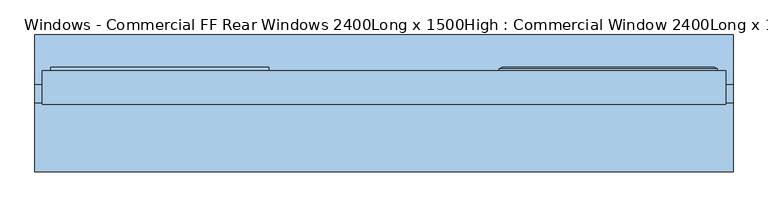
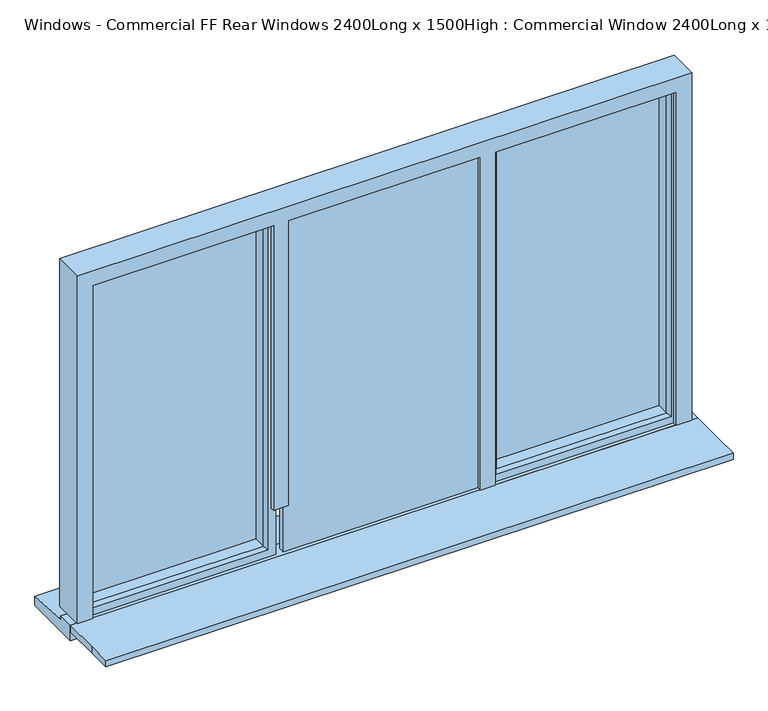
"""IFC4 building model written with IfcOpenShell, lengths in millimetres: window geometry, Windows - Commercial FF Rear Windows 2400Long x 1500High : Commercial Window 2400Long x 1500High."""

from ifc_helpers import new_model, si_unit, frame, origin, place, context, project, spatial, polyline, outline, extrude, faceted_brep, source, transform, mapped, element, save


def windows_commercial_ff_rear_windows_2400long_x_1500high_d88e899e(model_context):
    return source(origin(), model_context, "Body", "SolidModel", [
        extrude(outline(polyline([(-1860.0, -231.5434322), (-1860.0, -138.5434322), (-1860.0, 8.4565678), (590.0, 8.4565678), (590.0, -138.5434322), (590.0, -231.5434322), (-1860.0, -231.5434322)])), frame((0.0, 0.0, 636.5715519), z_axis=(0.0, 0.0, 1.0), x_axis=(1.0, 0.0, 0.0)), (0.0, 0.0, 1.0), 26.4284481),
        extrude(outline(polyline([(495.0, 87.4565678), (-190.0, 87.4565678), (-190.0, 111.4565678), (495.0, 111.4565678), (495.0, 87.4565678)])), frame((0.0, 0.0, 693.0), z_axis=(0.0, 0.0, 1.0), x_axis=(1.0, 0.0, 0.0)), (0.0, 0.0, 1.0), 1337.0),
        extrude(outline(polyline([(-1020.0, 47.4565678), (-250.0, 47.4565678), (-250.0, 23.4565678), (-1020.0, 23.4565678), (-1020.0, 47.4565678)])), frame((0.0, 0.0, 663.0), z_axis=(0.0, 0.0, 1.0), x_axis=(1.0, 0.0, 0.0)), (0.0, 0.0, 1.0), 1397.0),
        extrude(outline(polyline([(-1080.0, 87.4565678), (-1765.0, 87.4565678), (-1765.0, 111.4565678), (-1080.0, 111.4565678), (-1080.0, 87.4565678)])), frame((0.0, 0.0, 693.0), z_axis=(0.0, 0.0, 1.0), x_axis=(1.0, 0.0, 0.0)), (0.0, 0.0, 1.0), 1337.0),
        faceted_brep([(-1835.0, 5.4565678, 663.0), (-1775.0, 5.4565678, 663.0), (-1775.0, 5.4565678, 2040.0), (-1068.0, 5.4565678, 2040.0), (-1068.0, 5.4565678, 863.0), (-1010.0, 5.4565678, 863.0), (-1010.0, 5.4565678, 2040.0), (-260.0, 5.4565678, 2040.0), (-260.0, 5.4565678, 663.0), (-202.0, 5.4565678, 663.0), (-202.0, 5.4565678, 2040.0), (505.0, 5.4565678, 2040.0), (505.0, 5.4565678, 663.0), (565.0, 5.4565678, 663.0), (565.0, 5.4565678, 2100.0), (-1835.0, 5.4565678, 2100.0), (-1835.0, 123.4565678, 2100.0), (-1835.0, 123.4565678, 663.0), (-1835.0, 73.4565678, 663.0), (-1835.0, 8.4565678, 663.0), (-1795.0, 123.4565678, 663.0), (565.0, 123.4565678, 2100.0), (565.0, 123.4565678, 663.0), (525.0, 123.4565678, 663.0), (525.0, 123.4565678, 2060.0), (-220.0, 123.4565678, 2060.0), (-220.0, 123.4565678, 663.0), (-260.0, 123.4565678, 663.0), (-260.0, 123.4565678, 2060.0), (-1010.0, 123.4565678, 2060.0), (-1010.0, 123.4565678, 863.0), (-1050.0, 123.4565678, 863.0), (-1050.0, 123.4565678, 2060.0), (-1795.0, 123.4565678, 2060.0), (-1795.0, 23.4565678, 2060.0), (-1795.0, 23.4565678, 663.0), (-1795.0, 73.4565678, 663.0), (-1050.0, 23.4565678, 2060.0), (-1050.0, 23.4565678, 863.0), (-1068.0, 23.4565678, 863.0), (-1068.0, 23.4565678, 2040.0), (-1775.0, 23.4565678, 2040.0), (-1775.0, 23.4565678, 663.0), (525.0, 23.4565678, 2060.0), (525.0, 23.4565678, 663.0), (505.0, 23.4565678, 663.0), (505.0, 23.4565678, 2040.0), (-202.0, 23.4565678, 2040.0), (-202.0, 23.4565678, 663.0), (-220.0, 23.4565678, 663.0), (-220.0, 23.4565678, 2060.0), (-1010.0, 23.4565678, 863.0), (-1020.0, 23.4565678, 863.0), (-1020.0, 23.4565678, 2060.0), (-250.0, 23.4565678, 2060.0), (-250.0, 23.4565678, 663.0), (-260.0, 23.4565678, 663.0), (-260.0, 23.4565678, 2040.0), (-1010.0, 23.4565678, 2040.0), (-1775.0, 8.4565678, 663.0), (-1010.0, 47.4565678, 2060.0), (-260.0, 47.4565678, 2060.0), (-250.0, 47.4565678, 2060.0), (-1020.0, 47.4565678, 2060.0), (565.0, 8.4565678, 663.0), (565.0, 73.4565678, 663.0), (525.0, 73.4565678, 663.0), (505.0, 8.4565678, 663.0), (-1010.0, 47.4565678, 863.0), (-1020.0, 47.4565678, 863.0), (-250.0, 47.4565678, 663.0), (-260.0, 47.4565678, 663.0), (-260.0, 73.4565678, 663.0), (-220.0, 73.4565678, 663.0), (-202.0, 8.4565678, 663.0), (-260.0, 8.4565678, 663.0), (590.0, 248.4565678, 600.0), (590.0, 8.4565678, 600.0), (-1860.0, 8.4565678, 600.0), (-1860.0, 248.4565678, 600.0), (590.0, 248.4565678, 637.0666405), (-1860.0, 248.4565678, 637.0666405), (590.0, 73.4565678, 649.0962075), (-1860.0, 73.4565678, 649.0962075), (590.0, 8.4565678, 663.0), (590.0, 73.4565678, 663.0), (-1860.0, 73.4565678, 663.0), (-1860.0, 8.4565678, 663.0)], [[[0, 1, 2, 3, 4, 5, 6, 7, 8, 9, 10, 11, 12, 13, 14, 15]], [[0, 15, 16, 17, 18, 19]], [[20, 17, 16, 21, 22, 23, 24, 25, 26, 27, 28, 29, 30, 31, 32, 33]], [[20, 33, 34, 35, 36]], [[35, 34, 37, 38, 39, 40, 41, 42]], [[43, 44, 45, 46, 47, 48, 49, 50]], [[51, 52, 53, 54, 55, 56, 57, 58]], [[2, 1, 59, 42, 41]], [[15, 14, 21, 16]], [[34, 33, 32, 37]], [[24, 43, 50, 25]], [[60, 29, 28, 61, 62, 54, 53, 63]], [[2, 41, 40, 3]], [[46, 11, 10, 47]], [[6, 58, 57, 7]], [[14, 13, 64, 65, 22, 21]], [[24, 23, 66, 44, 43]], [[12, 11, 46, 45, 67]], [[5, 51, 58, 6]], [[39, 4, 3, 40]], [[31, 38, 37, 32]], [[68, 30, 29, 60]], [[69, 68, 60, 63]], [[52, 69, 63, 53]], [[62, 70, 55, 54]], [[70, 62, 61, 71]], [[71, 61, 28, 27, 72]], [[26, 25, 50, 49, 73]], [[10, 9, 74, 48, 47]], [[8, 7, 57, 56, 75]], [[76, 77, 78, 79]], [[80, 76, 79, 81]], [[82, 80, 81, 83]], [[84, 85, 65, 64]], [[86, 87, 19, 18]], [[72, 36, 35, 42, 59, 75, 56, 55, 70, 71]], [[66, 73, 49, 48, 74, 67, 45, 44]], [[17, 20, 36, 18]], [[1, 0, 19, 59]], [[23, 22, 65, 66]], [[13, 12, 67, 64]], [[51, 5, 4, 39, 38, 31, 30, 68, 69, 52]], [[27, 26, 73, 72]], [[9, 8, 75, 74]], [[84, 77, 76, 80, 82, 85]], [[87, 86, 83, 81, 79, 78]], [[85, 82, 83, 86, 18, 36, 72, 73, 66, 65]], [[77, 84, 64, 67, 74, 75, 59, 19, 87, 78]]]),
        faceted_brep([(-1050.0, 23.4565678, 2060.0), (-1050.0, 93.4565678, 2060.0), (-1795.0, 93.4565678, 2060.0), (-1795.0, 23.4565678, 2060.0), (-1090.0, 37.9494677, 2020.0), (-1079.8519623, 23.4565678, 2030.1480377), (-1765.1480377, 23.4565678, 2030.1480377), (-1755.0, 37.9494677, 2020.0), (-1090.0, 87.4565678, 2020.0), (-1755.0, 87.4565678, 2020.0), (-1080.0, 111.4565678, 2030.0), (-1080.0, 87.4565678, 2030.0), (-1765.0, 87.4565678, 2030.0), (-1765.0, 111.4565678, 2030.0), (-1090.0, 129.2300705, 2020.0), (-1090.0, 111.4565678, 2020.0), (-1755.0, 111.4565678, 2020.0), (-1755.0, 129.2300705, 2020.0), (-1071.1854344, 135.0035732, 2038.8145656), (-1773.8145656, 135.0035732, 2038.8145656), (-1795.0, 93.4565678, 663.0), (-1795.0, 23.4565678, 663.0), (-1765.1480377, 23.4565678, 692.8519623), (-1755.0, 37.9494677, 703.0), (-1755.0, 87.4565678, 703.0), (-1765.0, 87.4565678, 693.0), (-1765.0, 111.4565678, 693.0), (-1755.0, 111.4565678, 703.0), (-1755.0, 129.2300705, 703.0), (-1773.8145656, 135.0035732, 684.1854344), (-1050.0, 93.4565678, 663.0), (-1050.0, 23.4565678, 663.0), (-1079.8519623, 23.4565678, 692.8519623), (-1090.0, 37.9494677, 703.0), (-1090.0, 87.4565678, 703.0), (-1080.0, 87.4565678, 693.0), (-1080.0, 111.4565678, 693.0), (-1090.0, 111.4565678, 703.0), (-1090.0, 129.2300705, 703.0), (-1071.1854344, 135.0035732, 684.1854344), (-1040.0, 135.0035732, 653.0), (-1805.0, 135.0035732, 653.0), (-1805.0, 135.0035732, 2070.0), (-1040.0, 135.0035732, 2070.0), (-1040.0, 93.4565678, 2070.0), (-1805.0, 93.4565678, 2070.0), (-1805.0, 93.4565678, 653.0), (-1040.0, 93.4565678, 653.0)], [[[0, 1, 2, 3]], [[4, 5, 6, 7]], [[8, 4, 7, 9]], [[10, 11, 12, 13]], [[14, 15, 16, 17]], [[18, 14, 17, 19]], [[3, 2, 20, 21]], [[7, 6, 22, 23]], [[9, 7, 23, 24]], [[13, 12, 25, 26]], [[17, 16, 27, 28]], [[19, 17, 28, 29]], [[21, 20, 30, 31]], [[0, 3, 21, 31], [32, 22, 6, 5]], [[23, 22, 32, 33]], [[24, 23, 33, 34]], [[35, 25, 12, 11], [8, 9, 24, 34]], [[26, 25, 35, 36]], [[10, 13, 26, 36], [37, 27, 16, 15]], [[28, 27, 37, 38]], [[29, 28, 38, 39]], [[40, 41, 42, 43], [18, 19, 29, 39]], [[30, 1, 0, 31]], [[33, 32, 5, 4]], [[34, 33, 4, 8]], [[36, 35, 11, 10]], [[38, 37, 15, 14]], [[39, 38, 14, 18]], [[44, 43, 42, 45]], [[45, 42, 41, 46]], [[46, 41, 40, 47]], [[47, 40, 43, 44]], [[45, 46, 47, 44], [1, 30, 20, 2]]]),
        faceted_brep([(-230.0, 87.4565678, 2070.0), (-230.0, 129.2300705, 2070.0), (-230.0, 129.2300705, 653.0), (-230.0, 87.4565678, 653.0), (-220.0, 23.4565678, 2060.0), (-220.0, 87.4565678, 2060.0), (-220.0, 87.4565678, 663.0), (-220.0, 23.4565678, 663.0), (-180.0, 37.9494677, 2020.0), (-190.1480377, 23.4565678, 2030.1480377), (-190.1480377, 23.4565678, 692.8519623), (-180.0, 37.9494677, 703.0), (-180.0, 87.4565678, 2020.0), (-180.0, 87.4565678, 703.0), (-190.0, 111.4565678, 2030.0), (-190.0, 87.4565678, 2030.0), (-190.0, 87.4565678, 693.0), (-190.0, 111.4565678, 693.0), (-180.0, 129.2300705, 2020.0), (-180.0, 111.4565678, 2020.0), (-180.0, 111.4565678, 703.0), (-180.0, 129.2300705, 703.0), (-197.4457548, 135.0035732, 2037.4457548), (-197.4457548, 135.0035732, 685.5542452), (-219.2153903, 135.0035732, 2059.2153903), (-219.2153903, 135.0035732, 663.7846097), (535.0, 129.2300705, 653.0), (535.0, 87.4565678, 653.0), (525.0, 87.4565678, 663.0), (525.0, 23.4565678, 663.0), (495.1480377, 23.4565678, 692.8519623), (485.0, 37.9494677, 703.0), (485.0, 87.4565678, 703.0), (495.0, 87.4565678, 693.0), (495.0, 111.4565678, 693.0), (485.0, 111.4565678, 703.0), (485.0, 129.2300705, 703.0), (502.4457548, 135.0035732, 685.5542452), (524.2153903, 135.0035732, 663.7846097), (535.0, 129.2300705, 2070.0), (535.0, 87.4565678, 2070.0), (525.0, 87.4565678, 2060.0), (525.0, 23.4565678, 2060.0), (495.1480377, 23.4565678, 2030.1480377), (485.0, 37.9494677, 2020.0), (485.0, 87.4565678, 2020.0), (495.0, 87.4565678, 2030.0), (495.0, 111.4565678, 2030.0), (485.0, 111.4565678, 2020.0), (485.0, 129.2300705, 2020.0), (502.4457548, 135.0035732, 2037.4457548), (524.2153903, 135.0035732, 2059.2153903)], [[[0, 1, 2, 3]], [[4, 5, 6, 7]], [[8, 9, 10, 11]], [[12, 8, 11, 13]], [[14, 15, 16, 17]], [[18, 19, 20, 21]], [[22, 18, 21, 23]], [[1, 24, 25, 2]], [[3, 2, 26, 27]], [[7, 6, 28, 29]], [[11, 10, 30, 31]], [[13, 11, 31, 32]], [[17, 16, 33, 34]], [[21, 20, 35, 36]], [[23, 21, 36, 37]], [[2, 25, 38, 26]], [[27, 26, 39, 40]], [[29, 28, 41, 42]], [[31, 30, 43, 44]], [[32, 31, 44, 45]], [[34, 33, 46, 47]], [[36, 35, 48, 49]], [[37, 36, 49, 50]], [[26, 38, 51, 39]], [[40, 39, 1, 0]], [[42, 41, 5, 4]], [[7, 29, 42, 4], [9, 43, 30, 10]], [[44, 43, 9, 8]], [[45, 44, 8, 12]], [[15, 46, 33, 16], [13, 32, 45, 12]], [[47, 46, 15, 14]], [[17, 34, 47, 14], [19, 48, 35, 20]], [[49, 48, 19, 18]], [[50, 49, 18, 22]], [[24, 51, 38, 25], [23, 37, 50, 22]], [[39, 51, 24, 1]], [[3, 27, 40, 0], [5, 41, 28, 6]]]),
    ])


if __name__ == "__main__":
    model = new_model("IFC4")
    model_context = context("Model", 3, world=origin())
    ifc_project = project(units=[si_unit("LENGTHUNIT", "METRE", prefix="MILLI")], contexts=[model_context])
    site = spatial("IfcSite", under=ifc_project)
    building = spatial("IfcBuilding", under=site)
    placement = place(None, origin())
    windows_commercial_ff_rear_windows_2400long_x_1500high_shape = windows_commercial_ff_rear_windows_2400long_x_1500high_d88e899e(model_context)
    element("IfcWindow", 1, ObjectType="Windows - Commercial FF Rear Windows 2400Long x 1500High : Commercial Window 2400Long x 1500High", at=placement, inside=building, context=model_context, shape_type="MappedRepresentation", body=[
        mapped(windows_commercial_ff_rear_windows_2400long_x_1500high_shape, transform((0.0, 0.0, 0.0), x_axis=(1.0, 0.0, 0.0), y_axis=(0.0, 1.0, 0.0), z_axis=(0.0, 0.0, 1.0))),
    ])
    save(model, "model.ifc")

# Revit data of these elements
# Type "Windows - Commercial FF Rear Windows 2400Long x 1500High : Commercial Window 2400Long x 1500High"
#   Type Mark = "45"
#   Operation = "TriplePanelVertical"
#   Description = "Double Glazed First Floor Window"
#   Manufacturer = "aluminium Co"
#   Keynote = "L10"
#   Wrap Layers (Ext) from Ext = 100 mm
#   Wrap Layers (Int) from Ext = 177.5 mm
#   Window Board Projection = 25 mm
#   Window Board Extension = 25 mm
#   Visual Light Transmittance = 0.9
#   Solar Heat Gain Coefficient = 0.78
#   Rough Width = 2400 mm
#   Rough Height = 1500 mm
#   Height = 1500 mm
#   Width = 2400 mm
#   Heat Transfer Coefficient (U) = 3.6886 W/(m²·K)
#   Glazing Thickness = 24 mm
#   FrameOffset - External = 100 mm
#   Frame Depth = 100 mm
#   Default Head Height = 2500 mm
#   Cill Depth = 125 mm
#   Cavity Closer Width = 75 mm
#   Cavity Closer Offset from Ext = 115 mm
#   Cavity Closer Depth = 100 mm
#   Vis - Cavity Closers = yes
#   Define Thermal Properties by = 1
#   Material Trim = Window Frame
#   Material Glass = Glass
#   Material Frame = Window Frame
#   Construction Type Id = ""
#   Wall Closure = (empty or 0)
#   Analytic Construction = (empty or 0)
# Element 1 (IfcWindow, "Windows - Commercial FF Rear Windows 2400Long x 1500High : Commercial Window 2400Long x 1500High")
#   Materials on its faces: "Window Frame", "Glass"
# Materials
#   "Window Frame": class "Miscellaneous", colour RGB 249 249 249, transparency 0, Keynote = "L10"
#   "Glass": class "Glass", colour RGB 0 128 192, transparency 0.9, Description = "Soda Lime Glass", Cost = 0
